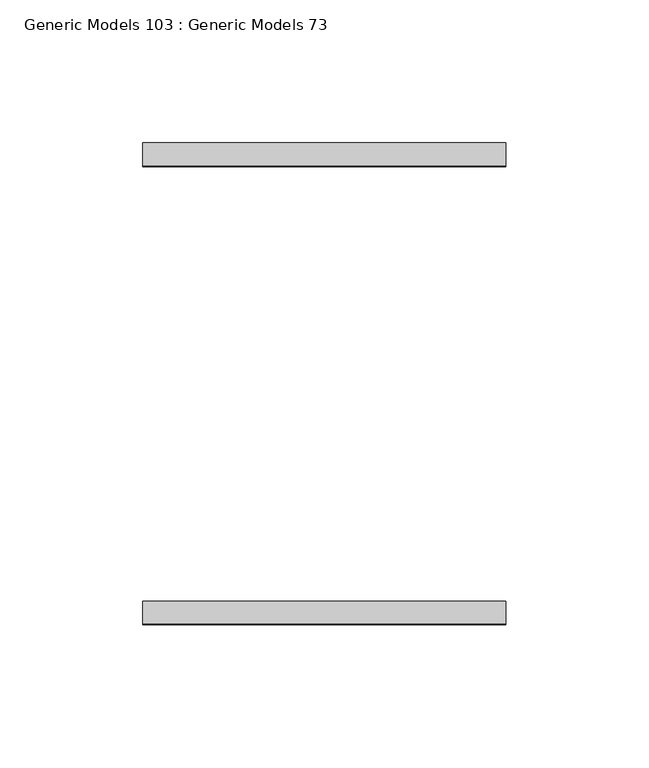
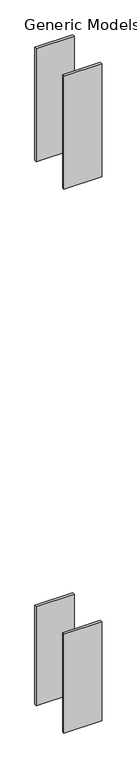
"""IFC4 building model written with IfcOpenShell, lengths in millimetres: proxy geometry, Generic Models 103 : Generic Models 73."""

from ifc_helpers import new_model, si_unit, frame, origin, place, context, project, spatial, polyline, outline, extrude, source, transform, mapped, element, save


def generic_models_103_generic_models_73_c6e0ad0c(model_context):
    return source(origin(), model_context, "Body", "SweptSolid", [
        extrude(outline(polyline([(32053.2090778, 30858.4781612), (32053.2090778, 30850.5406612), (31926.2090778, 30850.5406612), (31926.2090778, 30858.4781612), (32053.2090778, 30858.4781612)])), frame((0.0, 0.0, 268349.4125), z_axis=(0.0, 0.0, 1.0), x_axis=(1.0, 0.0, 0.0)), (0.0, 0.0, 1.0), 400.05),
        extrude(outline(polyline([(32053.2090778, 30698.1406612), (32053.2090778, 30690.2031612), (31926.2090778, 30690.2031612), (31926.2090778, 30698.1406612), (32053.2090778, 30698.1406612)])), frame((0.0, 0.0, 268349.4125), z_axis=(0.0, 0.0, 1.0), x_axis=(1.0, 0.0, 0.0)), (0.0, 0.0, 1.0), 400.05),
        extrude(outline(polyline([(32053.2090778, 30858.4781612), (32053.2090778, 30850.5406612), (31926.2090778, 30850.5406612), (31926.2090778, 30858.4781612), (32053.2090778, 30858.4781612)])), frame((0.0, 0.0, 266422.1875), z_axis=(0.0, 0.0, 1.0), x_axis=(1.0, 0.0, 0.0)), (0.0, 0.0, 1.0), 350.0376684),
        extrude(outline(polyline([(32053.2090778, 30698.1406612), (32053.2090778, 30690.2031612), (31926.2090778, 30690.2031612), (31926.2090778, 30698.1406612), (32053.2090778, 30698.1406612)])), frame((0.0, 0.0, 266422.1875), z_axis=(0.0, 0.0, 1.0), x_axis=(1.0, 0.0, 0.0)), (0.0, 0.0, 1.0), 350.0376684),
    ])


if __name__ == "__main__":
    model = new_model("IFC4")
    model_context = context("Model", 3, world=origin())
    ifc_project = project(units=[si_unit("LENGTHUNIT", "METRE", prefix="MILLI")], contexts=[model_context])
    site = spatial("IfcSite", under=ifc_project)
    building = spatial("IfcBuilding", under=site)
    placement = place(None, origin())
    generic_models_103_generic_models_73_shape = generic_models_103_generic_models_73_c6e0ad0c(model_context)
    element("IfcBuildingElementProxy", 1, Name="Generic Models 103 : Generic Models 73", ObjectType="Generic Models 103 : Generic Models 73", at=placement, inside=building, context=model_context, shape_type="MappedRepresentation", body=[
        mapped(generic_models_103_generic_models_73_shape, transform((0.0, 0.0, 0.0), x_axis=(1.0, 0.0, 0.0), y_axis=(0.0, 1.0, 0.0), z_axis=(0.0, 0.0, 1.0))),
    ])
    save(model, "model.ifc")

# Revit data of these elements
# Element 1 (IfcBuildingElementProxy, "Generic Models 103 : Generic Models 73")
#   Materials on its faces: "5/16 THICK GALV. SADDLE"
# Materials
#   "5/16 THICK GALV. SADDLE": class "Metal", colour RGB 199 199 199, transparency 0, Description = "Carbon steel", Cost = 0
